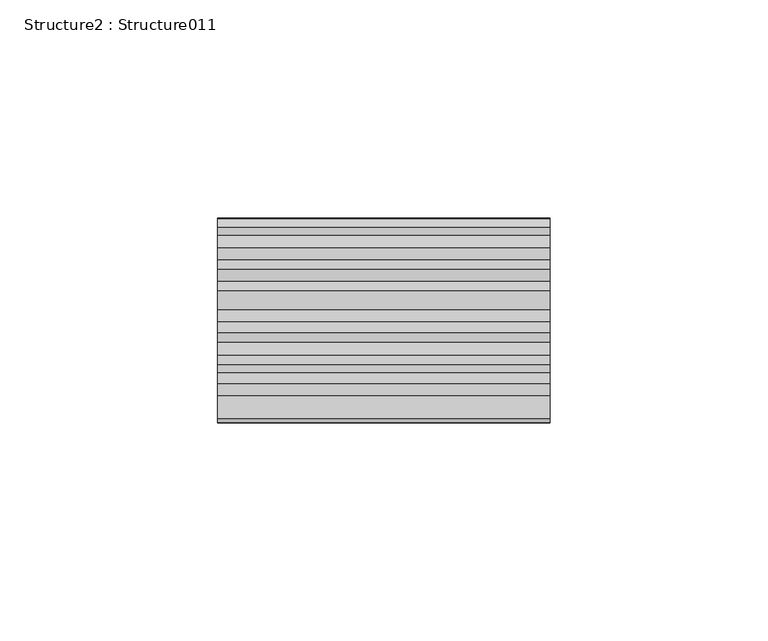
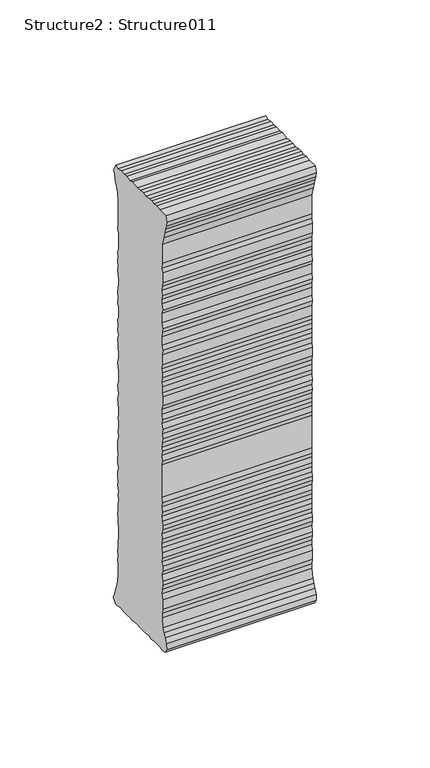
"""IFC4 building model written with IfcOpenShell, lengths in millimetres: proxy geometry, Structure2 : Structure011."""

from ifc_helpers import new_model, si_unit, frame, origin, place, context, project, spatial, polyline, outline, extrude, source, transform, mapped, element, save


def structure2_structure011_17c11ef0(model_context):
    return source(origin(), model_context, "Body", "SweptSolid", [
        extrude(outline(polyline([(4.3412703, 0.0), (7.4929278, 0.6976856), (10.0583012, 1.7563381), (12.8717356, 2.1701775), (15.4269694, 3.229564), (17.7464403, 0.8914403), (17.5897234, -1.2733707), (16.7650712, -4.0056411), (17.2545744, -5.9029569), (17.0538153, -8.6761457), (16.5685369, -11.1204062), (16.718605, -13.3065768), (16.2333879, -15.7499923), (15.7598686, -17.8910197), (15.8984835, -20.3761986), (15.4959253, -25.9369408), (15.0008132, -28.3762423), (15.4903776, -30.2727131), (14.6656641, -33.0058284), (14.8484435, -34.8809396), (14.6247457, -37.9709919), (14.7532821, -40.4545917), (14.3124742, -42.2845595), (12.03162, -43.6721405), (8.9781979, -43.1419138), (6.6012854, -41.7263244), (4.4997695, -40.6483464), (2.4082823, -39.5609016), (-2.4759526, -38.5898059), (-4.9415726, -38.4113126), (-7.4395981, -38.5396539), (-12.3674583, -38.182912), (-15.1197748, -37.3653026), (-17.9110045, -37.4724181), (-20.0921666, -37.6236981), (-22.2510629, -37.4674094), (-25.2923588, -36.6288799), (-27.8033554, -37.0654629), (-30.2782701, -36.8862967), (-32.3791153, -36.1158492), (-34.5746419, -36.2660894), (-37.3436059, -36.0656362), (-39.7878051, -35.5795128), (-42.2627199, -35.4003466), (-44.7472259, -35.5296668), (-47.4981489, -35.0213389), (-50.0184402, -35.457249), (-52.1773365, -35.3009603), (-54.313967, -34.8371029), (-56.7539413, -34.3512854), (-59.2426721, -34.4802997), (-62.0121845, -33.9706261), (-64.1840519, -34.122579), (-66.9442697, -33.6135782), (-84.5348382, -32.3401463), (-86.4084314, -32.5136922), (-89.4762179, -31.9824256), (-91.959879, -32.111807), (-93.7948554, -31.669787), (-96.5860853, -31.7769026), (-98.7672472, -31.9281826), (-101.2207412, -31.4413865), (-104.011971, -31.5485019), (-106.7406283, -30.7326053), (-108.931085, -30.8832125), (-111.6777832, -30.3751904), (-114.1526979, -30.1960242), (-116.6636946, -30.6326072), (-121.2983505, -30.2970912), (-123.4265313, -29.8338454), (-126.5115138, -29.6105147), (-128.6489893, -29.146596), (-131.4537386, -29.2527328), (-133.9159788, -29.0744841), (-136.0526093, -28.6106266), (-138.2329264, -28.7619679), (-143.7995833, -28.3589816), (-146.2731047, -28.4890968), (-148.7051778, -27.6946708), (-153.0364898, -27.3811146), (-155.8285646, -27.488169), (-157.9962071, -27.6404277), (-160.7476785, -26.8228795), (-165.6755388, -26.4661375), (-167.8798117, -26.9249251), (-170.9202626, -26.0864568), (-173.3858826, -25.9079635), (-175.2603209, -26.0814482), (-178.0078641, -25.573365), (-180.5101144, -25.7014006), (-182.6912765, -25.8526806), (-187.9351553, -25.4730611), (-190.0495199, -24.7016348), (-192.8542692, -24.8077717), (-203.0268532, -24.071349), (-207.4491019, -24.9904806), (-210.5921988, -25.6989787), (-212.7831334, -25.8444549), (-215.0000829, -26.6191501), (-217.5059485, -27.0552552), (-220.5382535, -25.9047984), (-220.1585728, -20.6600746), (-220.2650766, -17.8603952), (-219.7786475, -15.4119711), (-219.9523769, -13.5409127), (-219.7958435, -11.3786365), (-218.9627508, -8.3420435), (-219.4164687, -6.1381377), (-218.9299784, -3.6888686), (-218.4267203, -0.9375785), (-218.7239048, 3.4286034), (-217.9575483, 5.5433351), (-218.3664287, 8.3666033), (-217.9026324, 10.5023889), (-218.0090139, 13.3037582), (-217.19782, 16.0378524), (-217.6738037, 17.9341893), (-214.1331708, 19.5346555), (-212.3573351, 18.4751581), (-209.2949853, 17.9391887), (-204.5452515, 15.1218966), (-199.6256595, 14.451476), (-187.904247, 13.6029293), (-185.0982857, 13.7140747), (-182.9850718, 12.9384847), (-174.9578646, 12.3573721), (-172.4457171, 12.7981189), (-170.0077997, 12.3073539), (-167.8254257, 12.4636427), (-165.065575, 11.949572), (-162.8832009, 12.1058608), (-160.4393687, 11.6146677), (-158.301832, 11.1515939), (-155.8269173, 10.9724278), (-150.8542196, 11.2350482), (-148.0943689, 10.7209776), (-145.3019271, 10.8331018), (-143.1751937, 10.0565331), (-137.9439896, 9.6778311), (-136.0427548, 10.1628037), (-132.9804051, 9.6268343), (-130.4904623, 9.7608572), (-128.3679538, 8.9845944), (-125.8566513, 9.4254023), (-123.1103201, 8.9123104), (-120.9514239, 8.7560217), (-118.5063184, 8.2706822), (-116.0314037, 8.091516), (-113.2040827, 8.5094465), (-108.9302827, 7.5774454), (-103.3788351, 7.1755601), (-100.8726025, 7.6167351), (-99.037993, 7.1696454), (-96.5844379, 6.6836942), (-94.0782053, 7.1248691), (-91.0251502, 6.5895726), (-88.5715952, 6.1036214), (-86.1051302, 5.9250669), (-83.6164604, 6.0532362), (-81.1637503, 5.5673462), (-78.7015102, 5.3890976), (-76.2043908, 5.5166552), (-73.7601304, 5.0313768), (-71.2488279, 5.4721848), (-66.9301904, 5.1595462), (-64.1745645, 4.6457814), (-61.9930355, 4.8021314), (-59.2198466, 4.6013722), (-57.0964931, 3.8250482), (-54.2826917, 4.2439574), (-51.8162266, 4.0654029), (-49.6655987, 3.5954356), (-47.1815706, 3.7298868), (-44.4439245, 2.9090923), (-42.2619787, 3.0594663), (-39.8177182, 2.5741879), (-37.3341184, 2.7027243), (-34.249136, 2.4793935), (-32.0667619, 2.6356823), (-29.6094101, 2.1435104), (-26.8404462, 1.9430571), (-25.0113233, 1.5023104), (-19.4590308, 1.100364), (-17.5804289, 1.2726978), (-14.4954464, 1.0493671), (-12.0063486, 1.1834512), (-9.5532216, 0.6915852), (-7.6877111, 0.8708126), (-4.6253614, 0.3348432), (0.0, 0.0), (4.3412703, 0.0)])), frame((-35624.0862846, 275749.1590574, 4000.1487179), z_axis=(1.0, 0.0, 1.354250045437766e-12), x_axis=(1.3520748079695175e-12, 0.07220392475299618, -0.9973898902887796)), (0.0, 0.0, 1.0), 76.2),
    ])


if __name__ == "__main__":
    model = new_model("IFC4")
    model_context = context("Model", 3, world=origin())
    ifc_project = project(units=[si_unit("LENGTHUNIT", "METRE", prefix="MILLI")], contexts=[model_context])
    site = spatial("IfcSite", under=ifc_project)
    building = spatial("IfcBuilding", under=site)
    placement = place(None, origin())
    structure2_structure011_shape = structure2_structure011_17c11ef0(model_context)
    element("IfcBuildingElementProxy", 1, Name="Structure2 : Structure011", ObjectType="Structure2 : Structure011", at=placement, inside=building, context=model_context, shape_type="MappedRepresentation", body=[
        mapped(structure2_structure011_shape, transform((0.0, 0.0, 0.0), x_axis=(1.0, 0.0, 0.0), y_axis=(0.0, 1.0, 0.0), z_axis=(0.0, 0.0, 1.0))),
    ])
    save(model, "model.ifc")

# Revit data of these elements
# Type "Structure2 : Structure011"
#   NameOverride = "Structure011"
# Element 1 (IfcBuildingElementProxy, "Structure2 : Structure011")
#   Materials on its faces: "BRUSHED ALUMINUM LETTERING"
# Materials
#   "BRUSHED ALUMINUM LETTERING": class "Unassigned", colour RGB 169 181 186, transparency 0, Cost = 0
